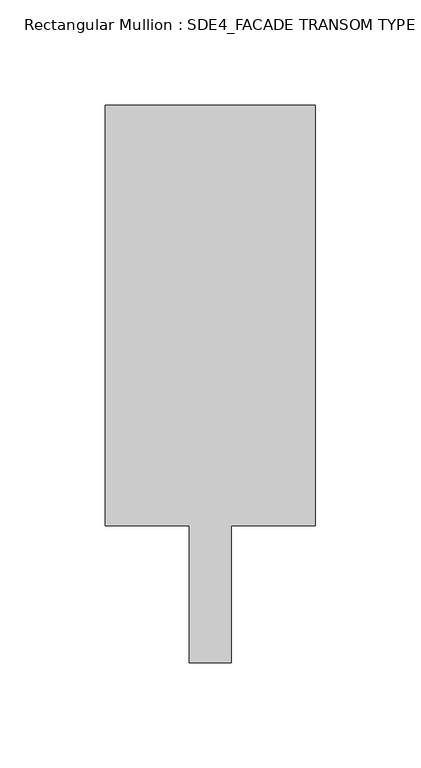
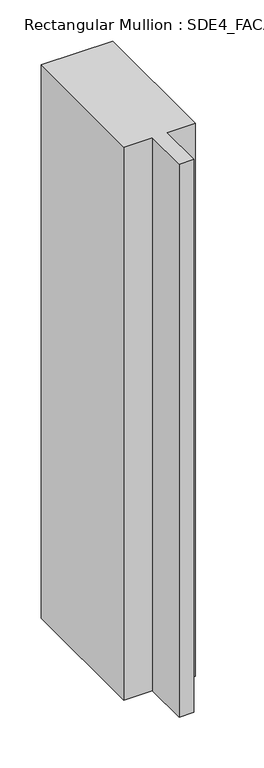
"""IFC4 building model written with IfcOpenShell, lengths in millimetres: member geometry, Rectangular Mullion : SDE4_FACADE TRANSOM TYPE 2."""

import ifcopenshell
import ifcopenshell.guid

model = None  # the IFC model being written
_history = None  # IfcOwnerHistory: only IFC2X3 demands one
_inside = {}  # id of a spatial element -> (the spatial element, [elements in it])
_under = {}  # id of a project, library or spatial element -> (it, [spatial elements below it])
_declared = {}  # id of a project -> (the project, [libraries it declares])
_typed = {}  # id of a type object -> (the type object, [elements of that type])
_made_of = {}  # id of a material, layer set ... -> (it, [elements and type objects made of it])


def new_model(schema):
    """Start an empty IFC model of exactly this schema.

    Asked for "IFC4X3", IfcOpenShell would pick the latest addendum, in which some entities
    have other attributes; the version numbers below select the first issue.
    IFC2X3 requires an IfcOwnerHistory on every rooted entity: one is made here for all.
    """
    global model, _history
    if schema == "IFC4X3":
        model = ifcopenshell.file(schema_version=(4, 3, 0, 0))
    else:
        model = ifcopenshell.file(schema=schema)
    _inside.clear()
    _under.clear()
    _declared.clear()
    _typed.clear()
    _made_of.clear()
    _history = None
    if model.schema == "IFC2X3":
        org = make("IfcOrganization", Name="unknown")
        user = make(
            "IfcPersonAndOrganization",
            ThePerson=make("IfcPerson", FamilyName="unknown"),
            TheOrganization=org,
        )
        app = make(
            "IfcApplication",
            ApplicationDeveloper=org,
            Version="unknown",
            ApplicationFullName="unknown",
            ApplicationIdentifier="unknown",
        )
        _history = make(
            "IfcOwnerHistory",
            OwningUser=user,
            OwningApplication=app,
            ChangeAction="ADDED",
            CreationDate=0,
        )
    return model


def make(cls, **values):
    """One entity of the class cls with the attributes given. An attribute that is None is left unset."""
    return model.create_entity(
        cls, **{name: value for name, value in values.items() if value is not None}
    )


def rooted(cls, **values):
    """An entity with a GlobalId (a new one), such as an element, a storey or a relation."""
    return make(cls, GlobalId=ifcopenshell.guid.new(), OwnerHistory=_history, **values)


def si_unit(unit_type, name, prefix=None):
    """IfcSIUnit, for example si_unit("LENGTHUNIT", "METRE", prefix="MILLI")."""
    return make("IfcSIUnit", UnitType=unit_type, Prefix=prefix, Name=name)


def assignment(units):
    """IfcUnitAssignment: the units of a project."""
    return None if units is None else make("IfcUnitAssignment", Units=units)


def point(xyz):
    """IfcCartesianPoint."""
    return None if xyz is None else make("IfcCartesianPoint", Coordinates=xyz)


def direction(xyz):
    """IfcDirection."""
    return None if xyz is None else make("IfcDirection", DirectionRatios=xyz)


def frame(location, z_axis=None, x_axis=None):
    """IfcAxis2Placement3D, a coordinate frame: its origin and axes. An axis left out is left unset."""
    return make(
        "IfcAxis2Placement3D",
        Location=point(location),
        Axis=direction(z_axis),
        RefDirection=direction(x_axis),
    )


def origin():
    """The frame at (0, 0, 0) with its axes left unset."""
    return frame((0.0, 0.0, 0.0))


def place(relative_to, where):
    """IfcLocalPlacement: puts the frame where relative to a parent placement (None: the world)."""
    return make(
        "IfcLocalPlacement", PlacementRelTo=relative_to, RelativePlacement=where
    )


def context(
    kind, dimensions, precision=None, world=None, true_north=None, identifier=None
):
    """IfcGeometricRepresentationContext, for example the 3D "Model" context."""
    return make(
        "IfcGeometricRepresentationContext",
        ContextIdentifier=identifier,
        ContextType=kind,
        CoordinateSpaceDimension=dimensions,
        Precision=precision,
        WorldCoordinateSystem=world,
        TrueNorth=true_north,
    )


def project(units=None, contexts=None):
    """IfcProject with its units and contexts."""
    return rooted(
        "IfcProject",
        Name="project",
        RepresentationContexts=contexts,
        UnitsInContext=assignment(units),
    )


def spatial(cls, under=None, at=None, **own):
    """A site, building, storey or space (cls), placed at a placement, below another one or the project."""
    s = rooted(cls, ObjectPlacement=at, **own)
    if under is not None:
        _under.setdefault(under.id(), (under, []))[1].append(s)
    return s


def polyline(points):
    """IfcPolyline through the points."""
    return make("IfcPolyline", Points=[point(p) for p in points])


def outline(outer, holes=None, kind="AREA"):
    """IfcArbitraryClosedProfileDef: a profile drawn as a closed curve; with holes, ...WithVoids."""
    if holes is None:
        return make("IfcArbitraryClosedProfileDef", ProfileType=kind, OuterCurve=outer)
    return make(
        "IfcArbitraryProfileDefWithVoids",
        ProfileType=kind,
        OuterCurve=outer,
        InnerCurves=holes,
    )


def extrude(swept, where, along, depth):
    """IfcExtrudedAreaSolid: the profile swept, set in the frame where, extruded along a direction by depth."""
    return make(
        "IfcExtrudedAreaSolid",
        SweptArea=swept,
        Position=where,
        ExtrudedDirection=direction(along),
        Depth=depth,
    )


def shape(context_of_items, identifier, shape_type, items):
    """IfcShapeRepresentation: the items that make up one representation, for example the "Body"."""
    return make(
        "IfcShapeRepresentation",
        ContextOfItems=context_of_items,
        RepresentationIdentifier=identifier,
        RepresentationType=shape_type,
        Items=items,
    )


def source(mapping_origin, context_of_items, identifier, shape_type, items):
    """IfcRepresentationMap: a shape defined once, which mapped items show again and again."""
    return make(
        "IfcRepresentationMap",
        MappingOrigin=mapping_origin,
        MappedRepresentation=shape(context_of_items, identifier, shape_type, items),
    )


def transform(
    local_origin,
    x_axis=None,
    y_axis=None,
    z_axis=None,
    scale=None,
    scale2=None,
    scale3=None,
    uniform=True,
):
    """IfcCartesianTransformationOperator3D, or its non-uniform kind. x_axis, y_axis, z_axis: its Axis1, 2, 3."""
    if uniform:
        return make(
            "IfcCartesianTransformationOperator3D",
            Axis1=direction(x_axis),
            Axis2=direction(y_axis),
            LocalOrigin=point(local_origin),
            Scale=scale,
            Axis3=direction(z_axis),
        )
    return make(
        "IfcCartesianTransformationOperator3DnonUniform",
        Axis1=direction(x_axis),
        Axis2=direction(y_axis),
        LocalOrigin=point(local_origin),
        Scale=scale,
        Axis3=direction(z_axis),
        Scale2=scale2,
        Scale3=scale3,
    )


def mapped(mapping_source, mapping_target):
    """IfcMappedItem: shows the shape of a source again, moved by a transform."""
    return make(
        "IfcMappedItem", MappingSource=mapping_source, MappingTarget=mapping_target
    )


def made_of(thing, what):
    """Note that an element or type object is made of a material, layer set ...; save() writes the relation."""
    if what is not None:
        _made_of.setdefault(what.id(), (what, []))[1].append(thing)
    return thing


def element(
    cls,
    number,
    at=None,
    inside=None,
    cuts=None,
    type_object=None,
    material=None,
    context=None,
    identifier="Body",
    shape_type=None,
    held_by="IfcProductDefinitionShape",
    body=None,
    shapes=None,
    **own,
):
    """One element of the class cls, such as IfcWall. Its Tag is "e" and its number.

    at: its placement. inside: the storey or other place that contains it. cuts: it is an
    opening in that element (IfcRelVoidsElement). A single representation is given by context,
    identifier, shape_type and body (its items); several are given by shapes. held_by: the class
    of the entity that holds the representations. save() writes the other relations.
    """
    e = rooted(cls, Tag="e%d" % number, ObjectPlacement=at, **own)
    if body is not None:
        shapes = [shape(context, identifier, shape_type, body)]
    if shapes is not None:
        e.Representation = make(held_by, Representations=shapes)
    if inside is not None:
        _inside.setdefault(inside.id(), (inside, []))[1].append(e)
    if cuts is not None:
        rooted(
            "IfcRelVoidsElement", RelatingBuildingElement=cuts, RelatedOpeningElement=e
        )
    if type_object is not None:
        _typed.setdefault(type_object.id(), (type_object, []))[1].append(e)
    return made_of(e, material)


def aggregate(whole, parts):
    """IfcRelAggregates: a whole, such as a stair, and the parts it consists of."""
    return rooted("IfcRelAggregates", RelatingObject=whole, RelatedObjects=parts)


def save(model, path):
    """Write the relations noted so far, then the file.

    IfcRelAggregates (storeys below a building ...), IfcRelContainedInSpatialStructure (elements
    in a storey), IfcRelDefinesByType, IfcRelAssociatesMaterial and IfcRelDeclares: one each for
    every whole, place, type object, material and project.
    """
    for whole, parts in _under.values():
        aggregate(whole, parts)
    for where, things in _inside.values():
        rooted(
            "IfcRelContainedInSpatialStructure",
            RelatedElements=things,
            RelatingStructure=where,
        )
    for kind, things in _typed.values():
        rooted("IfcRelDefinesByType", RelatedObjects=things, RelatingType=kind)
    for what, things in _made_of.values():
        rooted("IfcRelAssociatesMaterial", RelatedObjects=things, RelatingMaterial=what)
    for by, libraries in _declared.values():
        rooted("IfcRelDeclares", RelatingContext=by, RelatedDefinitions=libraries)
    model.write(path)


def rectangular_mullion_sde4_facade_transom_type_2_33d0c89e(model_context):
    return source(origin(), model_context, "Body", "SweptSolid", [
        extrude(outline(polyline([(50.0, 132.5), (50.0, -67.5), (10.0, -67.5), (10.0, -132.5), (-10.0, -132.5), (-10.0, -67.5), (-50.0, -67.5), (-50.0, 132.5), (50.0, 132.5)])), frame((0.0, 0.0, -817.5), z_axis=(0.0, 0.0, 1.0), x_axis=(1.0, 0.0, 0.0)), (0.0, 0.0, 1.0), 817.5),
    ])


if __name__ == "__main__":
    model = new_model("IFC4")
    model_context = context("Model", 3, world=origin())
    ifc_project = project(units=[si_unit("LENGTHUNIT", "METRE", prefix="MILLI")], contexts=[model_context])
    site = spatial("IfcSite", under=ifc_project)
    building = spatial("IfcBuilding", under=site)
    placement = place(None, origin())
    rectangular_mullion_sde4_facade_transom_type_2_shape = rectangular_mullion_sde4_facade_transom_type_2_33d0c89e(model_context)
    element("IfcMember", 1, ObjectType="Rectangular Mullion : SDE4_FACADE TRANSOM TYPE 2", at=placement, inside=building, context=model_context, shape_type="MappedRepresentation", body=[
        mapped(rectangular_mullion_sde4_facade_transom_type_2_shape, transform((0.0, 0.0, 0.0), x_axis=(1.0, 0.0, 0.0), y_axis=(0.0, 1.0, 0.0), z_axis=(0.0, 0.0, 1.0))),
    ])
    save(model, "model.ifc")

# Revit data of these elements
# Type "Rectangular Mullion : SDE4_FACADE TRANSOM TYPE 2"
#   built-in parameter 1007322 = 0.869423 (stored number, unit not read)
#   built-in parameter 1007321 = 0.164042 (stored number, unit not read)
#   built-in parameter 1007320 = 0.164042 (stored number, unit not read)
